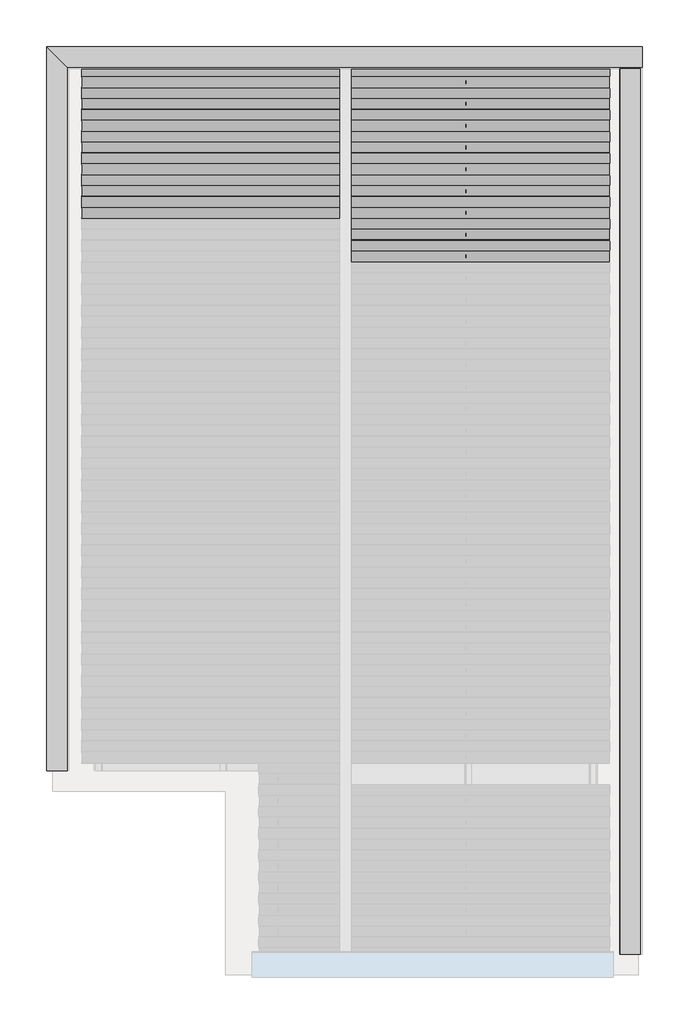
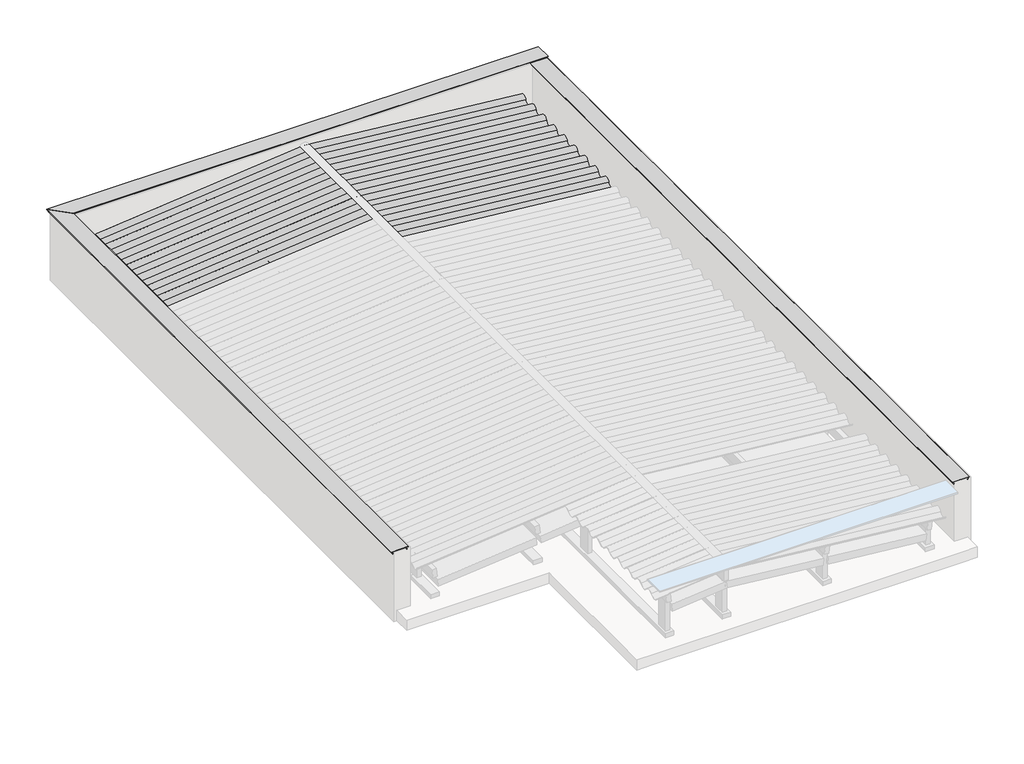
# One storey, part 4 of 4: 23 beams, 10 columns, 1 proxy.
# Revit data of these elements (continued)
# Elements 2, 4 (IfcBeam, "Madeira de lei : Berço 6x12cm")
#   Comments = ""
#   Uso = "TELHADOS ESTRUTURAS"
#   Compr Cmcl = 6.00 m
#   Structural Material = .MADEIRAMENTO
#   Phase Created = CC_AP
#   Materials on its faces: ".MADEIRAMENTO"
# Elements 8, 9, 10, 11, 12, 13, 14, 15, 16, 17, 18, 19, 20, 21, 22, 23 (IfcBeam, "Telha Ondulada : Fibrocimento")
#   Uso = "TELHADOS TELHAS"
#   Phase Created = CC_AP
#   Materials on its faces: ".TELHA DE FIBROCIMENTO"
# Element 24 (IfcBuildingElementProxy, ".CC_RUFO_PINGADEIRA_22 cm")
#   Uso = "TELHADOS RUFOS"
#   Nível de Ref. = "ESTAR/JANTAR/GALERIA"
#   Phase Created = CC_AP
#   Materials on its faces: ".ALUMÍNIO COM PINTURA LÁTEX BRANCA"
# Elements 25, 26, 31, 32, 33, 34 (IfcColumn, "Madeira de lei-Coluna : Pontalete 6X16cm")
#   Comments = ""
#   Uso = "TELHADOS ESTRUTURAS"
#   Compr Cmcl = 3.00 m
#   Structural Material = .MADEIRAMENTO
#   Phase Created = CC_AP
#   Materials on its faces: ".MADEIRAMENTO"
# Elements 27, 28, 29, 30 (IfcColumn, "Madeira de lei-Coluna : Pontalete 6X16cm")
#   Comments = ""
#   Uso = "TELHADOS ESTRUTURAS"
#   Compr Cmcl = 5.00 m
#   Structural Material = .MADEIRAMENTO
#   Phase Created = CC_AP
#   Materials on its faces: ".MADEIRAMENTO"
# Materials
#   ".TELHA DE FIBROCIMENTO": class "CC_TELHADO", colour RGB 77 77 76, transparency 0, Description = "TELHA ONDULADA FIBROCIMENTO", Cost = 0
#   ".MADEIRAMENTO": class ".CC_MADEIRAS", colour RGB 212 179 113, transparency 0, Cost = 0
#   ".ALUMÍNIO COM PINTURA LÁTEX BRANCA": class "Generic", colour RGB 250 250 250, transparency 0, Cost = 0
